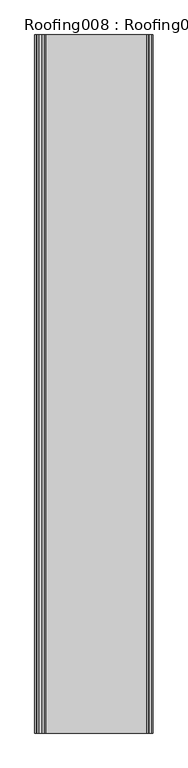
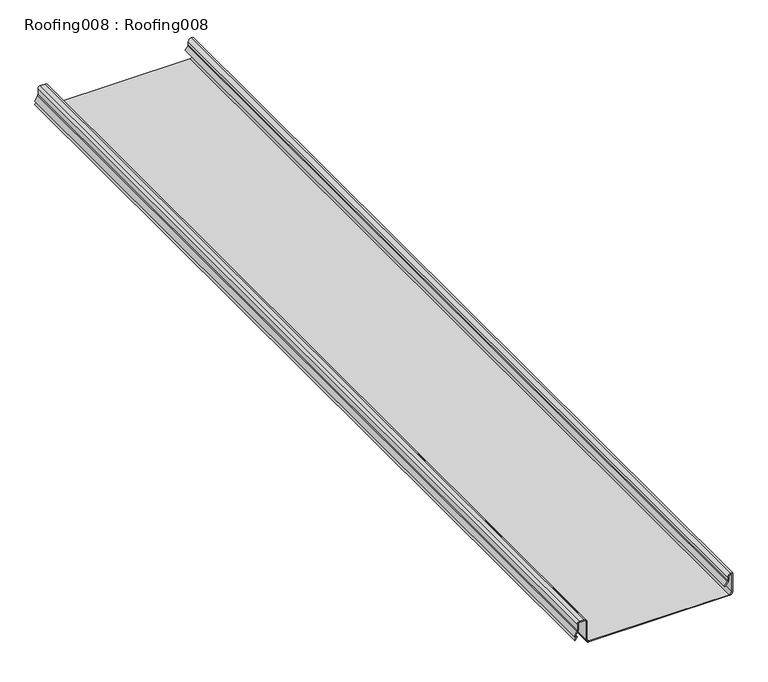
"""IFC4 building model written with IfcOpenShell, lengths in millimetres: proxy geometry, Roofing008 : Roofing008."""

from ifc_helpers import new_model, si_unit, point, frame, frame_2d, origin, place, context, project, spatial, polyline, circle_curve, trimmed, segment, composite_curve, outline, extrude, source, transform, mapped, element, save


def roofing008_roofing008_38f271d3(model_context):
    return source(origin(), model_context, "Body", "SweptSolid", [
        extrude(outline(composite_curve([segment(trimmed(circle_curve(frame_2d((42571.8416239, -541.7727869)), 5.08), [point((42568.8585944, -537.6608609))], [point((42571.8416239, -536.6927869))], False, "CARTESIAN"), True, "CONTINUOUS"), segment(polyline([(42571.8416239, -536.6927869), (42578.5981823, -536.6927869)]), True, "CONTINUOUS"), segment(trimmed(circle_curve(frame_2d((42578.5981823, -531.6127869)), 5.08), [point((42578.5981823, -536.6927869))], [point((42583.6781823, -531.6127869))], True, "CARTESIAN"), True, "CONTINUOUS"), segment(polyline([(42583.6781823, -531.6127869), (42583.6781823, -530.0179822), (42543.9409948, -530.0179822)]), True, "CONTINUOUS"), segment(trimmed(circle_curve(frame_2d((42543.9409948, -535.0979822)), 5.08), [point((42543.9409948, -530.0179822))], [point((42538.8609948, -535.0979822))], True, "CARTESIAN"), True, "CONTINUOUS"), segment(polyline([(42538.8609948, -535.0979822), (42538.8609948, -835.3720642)]), True, "CONTINUOUS"), segment(trimmed(circle_curve(frame_2d((42543.9409948, -835.3720642)), 5.08), [point((42538.8609948, -835.3720642))], [point((42543.9409948, -840.4520642))], True, "CARTESIAN"), True, "CONTINUOUS"), segment(polyline([(42543.9409948, -840.4520642), (42585.5544323, -840.4520642)]), True, "CONTINUOUS"), segment(trimmed(circle_curve(frame_2d((42585.5544323, -845.5320642)), 5.08), [point((42585.5544323, -840.4520642))], [point((42590.6344323, -845.5320642))], False, "CARTESIAN"), True, "CONTINUOUS"), segment(polyline([(42590.6344323, -845.5320642), (42590.6344323, -855.5398411)]), True, "CONTINUOUS"), segment(trimmed(circle_curve(frame_2d((42585.5544323, -855.5398411)), 5.08), [point((42590.6344323, -855.5398411))], [point((42585.5544323, -860.6198411))], False, "CARTESIAN"), True, "CONTINUOUS"), segment(polyline([(42585.5544323, -860.6198411), (42572.3718581, -860.6198411)]), True, "CONTINUOUS"), segment(trimmed(circle_curve(frame_2d((42572.3718581, -865.6998411)), 5.08), [point((42572.3718581, -860.6198411))], [point((42569.8678467, -861.2798494))], True, "CARTESIAN"), True, "CONTINUOUS"), segment(polyline([(42569.8678467, -861.2798494), (42559.3102135, -867.2609544), (42556.8688073, -863.0968919), (42551.2672448, -867.0959154), (42550.1051711, -865.4681608), (42557.4874863, -860.1978365), (42560.0388845, -864.5495013), (42568.8820154, -859.5396952)]), True, "CONTINUOUS"), segment(trimmed(circle_curve(frame_2d((42572.3718581, -865.6998411)), 7.08), [point((42568.8820154, -859.5396952))], [point((42572.3718581, -858.6198411))], False, "CARTESIAN"), True, "CONTINUOUS"), segment(polyline([(42572.3718581, -858.6198411), (42585.5544323, -858.6198411)]), True, "CONTINUOUS"), segment(trimmed(circle_curve(frame_2d((42585.5544323, -855.5398411)), 3.08), [point((42585.5544323, -858.6198411))], [point((42588.6344323, -855.5398411))], True, "CARTESIAN"), True, "CONTINUOUS"), segment(polyline([(42588.6344323, -855.5398411), (42588.6344323, -845.5320642)]), True, "CONTINUOUS"), segment(trimmed(circle_curve(frame_2d((42585.5544323, -845.5320642)), 3.08), [point((42588.6344323, -845.5320642))], [point((42585.5544323, -842.4520642))], True, "CARTESIAN"), True, "CONTINUOUS"), segment(polyline([(42585.5544323, -842.4520642), (42543.9409948, -842.4520642)]), True, "CONTINUOUS"), segment(trimmed(circle_curve(frame_2d((42543.9409948, -835.3720642)), 7.08), [point((42543.9409948, -842.4520642))], [point((42536.8609948, -835.3720642))], False, "CARTESIAN"), True, "CONTINUOUS"), segment(polyline([(42536.8609948, -835.3720642), (42536.8609948, -535.0979822)]), True, "CONTINUOUS"), segment(trimmed(circle_curve(frame_2d((42543.9409948, -535.0979822)), 7.08), [point((42536.8609948, -535.0979822))], [point((42543.9409948, -528.0179822))], False, "CARTESIAN"), True, "CONTINUOUS"), segment(polyline([(42543.9409948, -528.0179822), (42585.6781823, -528.0179822), (42585.6781823, -531.6127869)]), True, "CONTINUOUS"), segment(trimmed(circle_curve(frame_2d((42578.5981823, -531.6127869)), 7.08), [point((42585.6781823, -531.6127869))], [point((42578.5981823, -538.6927869))], False, "CARTESIAN"), True, "CONTINUOUS"), segment(polyline([(42578.5981823, -538.6927869), (42571.8416239, -538.6927869)]), True, "CONTINUOUS"), segment(trimmed(circle_curve(frame_2d((42571.8416239, -541.7727869)), 3.08), [point((42571.8416239, -538.6927869))], [point((42570.0330155, -539.2797294))], True, "CARTESIAN"), True, "CONTINUOUS"), segment(polyline([(42570.0330155, -539.2797294), (42561.5588533, -545.427378), (42560.3844323, -543.8085095), (42568.8585944, -537.6608609)]), True, "CONTINUOUS")], self_intersect=False)), frame((0.0, -1052.8906574, 0.0), z_axis=(0.0, 1.0, 0.0), x_axis=(0.0, 0.0, 1.0)), (0.0, 0.0, 1.0), 2000.0),
    ])


if __name__ == "__main__":
    model = new_model("IFC4")
    model_context = context("Model", 3, world=origin())
    ifc_project = project(units=[si_unit("LENGTHUNIT", "METRE", prefix="MILLI")], contexts=[model_context])
    site = spatial("IfcSite", under=ifc_project)
    building = spatial("IfcBuilding", under=site)
    placement = place(None, origin())
    roofing008_roofing008_shape = roofing008_roofing008_38f271d3(model_context)
    element("IfcBuildingElementProxy", 1, Name="Roofing008 : Roofing008", ObjectType="Roofing008 : Roofing008", at=placement, inside=building, context=model_context, shape_type="MappedRepresentation", body=[
        mapped(roofing008_roofing008_shape, transform((0.0, 0.0, 0.0), x_axis=(1.0, 0.0, 0.0), y_axis=(0.0, 1.0, 0.0), z_axis=(0.0, 0.0, 1.0))),
    ])
    save(model, "model.ifc")

# Revit data of these elements
# Type "Roofing008 : Roofing008"
#   NameOverride = "Roofing008"
# Element 1 (IfcBuildingElementProxy, "Roofing008 : Roofing008")
#   Materials on its faces: "STANDING SEAM METAL ROOF"
# Materials
#   "STANDING SEAM METAL ROOF": class "Unassigned", colour RGB 128 128 128, transparency 0
